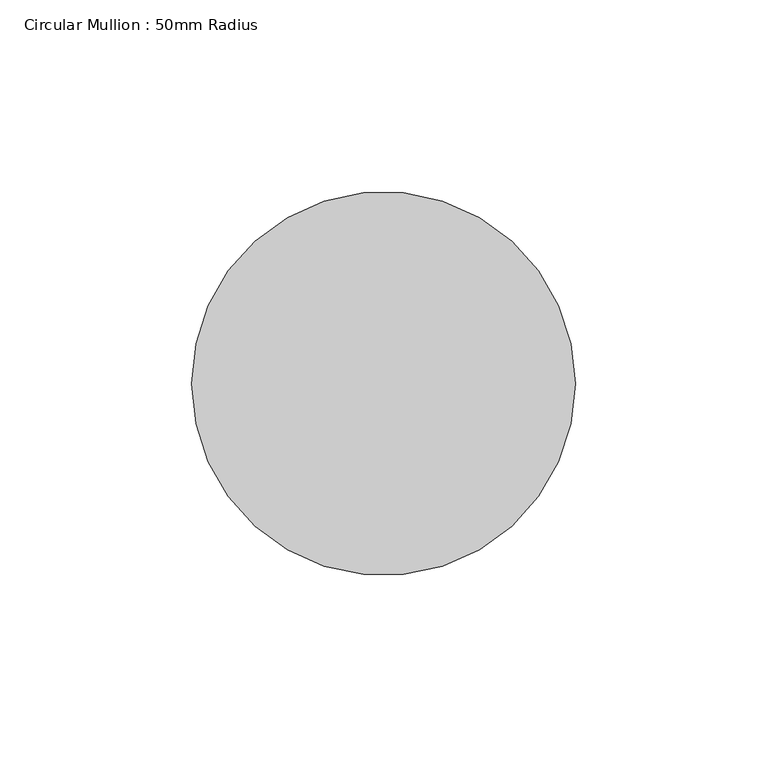
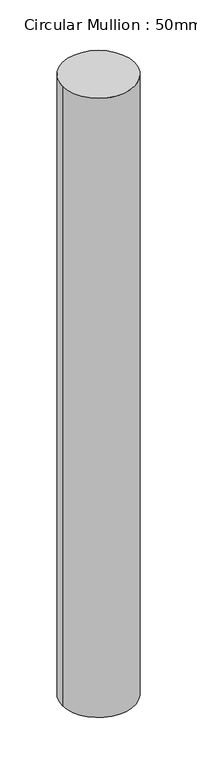
"""IFC4 building model written with IfcOpenShell, lengths in millimetres: member geometry, Circular Mullion : 50mm Radius."""

from ifc_helpers import new_model, si_unit, point, frame, origin, origin_2d, place, context, project, spatial, circle_curve, trimmed, segment, composite_curve, outline, extrude, source, transform, mapped, element, save


def circular_mullion_50mm_radius_b353e2a7(model_context):
    return source(origin(), model_context, "Body", "SweptSolid", [
        extrude(outline(composite_curve([segment(trimmed(circle_curve(origin_2d(), 50.0), [point((50.0, 0.0))], [point((-50.0, 0.0))], False, "CARTESIAN"), True, "CONTINUOUS"), segment(trimmed(circle_curve(origin_2d(), 50.0), [point((-50.0, 0.0))], [point((50.0, 0.0))], False, "CARTESIAN"), True, "CONTINUOUS")], self_intersect=False)), frame((0.0, 0.0, -906.1813672), z_axis=(0.0, 0.0, 1.0), x_axis=(1.0, 0.0, 0.0)), (0.0, 0.0, 1.0), 906.1813672),
    ])


if __name__ == "__main__":
    model = new_model("IFC4")
    model_context = context("Model", 3, world=origin())
    ifc_project = project(units=[si_unit("LENGTHUNIT", "METRE", prefix="MILLI")], contexts=[model_context])
    site = spatial("IfcSite", under=ifc_project)
    building = spatial("IfcBuilding", under=site)
    placement = place(None, origin())
    circular_mullion_50mm_radius_shape = circular_mullion_50mm_radius_b353e2a7(model_context)
    element("IfcMember", 1, ObjectType="Circular Mullion : 50mm Radius", at=placement, inside=building, context=model_context, shape_type="MappedRepresentation", body=[
        mapped(circular_mullion_50mm_radius_shape, transform((0.0, 0.0, 0.0), x_axis=(1.0, 0.0, 0.0), y_axis=(0.0, 1.0, 0.0), z_axis=(0.0, 0.0, 1.0))),
    ])
    save(model, "model.ifc")

# Revit data of these elements
# Type "Circular Mullion : 50mm Radius"
#   built-in parameter 1007350 = 0.164042 (stored number, unit not read)
# Element 1 (IfcMember, "Circular Mullion : 50mm Radius")
#   Materials on its faces: "Aluminium"
# Materials
#   "Aluminium": class "Metal", colour RGB 247 247 247, transparency 0, Description = "Aluminium 6061", Cost = 0
